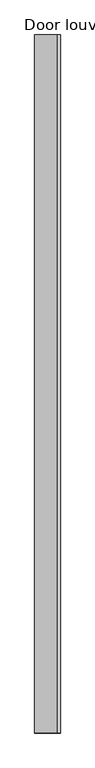
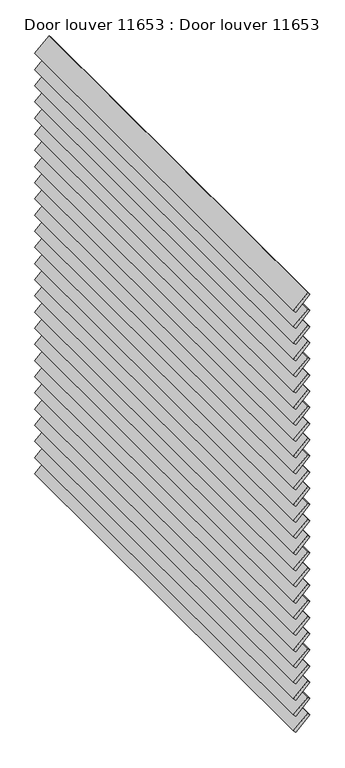
"""IFC4 building model written with IfcOpenShell, lengths in millimetres: proxy geometry, Door louver 11653 : Door louver 11653."""

import ifcopenshell
import ifcopenshell.guid

model = None  # the IFC model being written
_history = None  # IfcOwnerHistory: only IFC2X3 demands one
_inside = {}  # id of a spatial element -> (the spatial element, [elements in it])
_under = {}  # id of a project, library or spatial element -> (it, [spatial elements below it])
_declared = {}  # id of a project -> (the project, [libraries it declares])
_typed = {}  # id of a type object -> (the type object, [elements of that type])
_made_of = {}  # id of a material, layer set ... -> (it, [elements and type objects made of it])


def new_model(schema):
    """Start an empty IFC model of exactly this schema.

    Asked for "IFC4X3", IfcOpenShell would pick the latest addendum, in which some entities
    have other attributes; the version numbers below select the first issue.
    IFC2X3 requires an IfcOwnerHistory on every rooted entity: one is made here for all.
    """
    global model, _history
    if schema == "IFC4X3":
        model = ifcopenshell.file(schema_version=(4, 3, 0, 0))
    else:
        model = ifcopenshell.file(schema=schema)
    _inside.clear()
    _under.clear()
    _declared.clear()
    _typed.clear()
    _made_of.clear()
    _history = None
    if model.schema == "IFC2X3":
        org = make("IfcOrganization", Name="unknown")
        user = make(
            "IfcPersonAndOrganization",
            ThePerson=make("IfcPerson", FamilyName="unknown"),
            TheOrganization=org,
        )
        app = make(
            "IfcApplication",
            ApplicationDeveloper=org,
            Version="unknown",
            ApplicationFullName="unknown",
            ApplicationIdentifier="unknown",
        )
        _history = make(
            "IfcOwnerHistory",
            OwningUser=user,
            OwningApplication=app,
            ChangeAction="ADDED",
            CreationDate=0,
        )
    return model


def make(cls, **values):
    """One entity of the class cls with the attributes given. An attribute that is None is left unset."""
    return model.create_entity(
        cls, **{name: value for name, value in values.items() if value is not None}
    )


def rooted(cls, **values):
    """An entity with a GlobalId (a new one), such as an element, a storey or a relation."""
    return make(cls, GlobalId=ifcopenshell.guid.new(), OwnerHistory=_history, **values)


def si_unit(unit_type, name, prefix=None):
    """IfcSIUnit, for example si_unit("LENGTHUNIT", "METRE", prefix="MILLI")."""
    return make("IfcSIUnit", UnitType=unit_type, Prefix=prefix, Name=name)


def assignment(units):
    """IfcUnitAssignment: the units of a project."""
    return None if units is None else make("IfcUnitAssignment", Units=units)


def point(xyz):
    """IfcCartesianPoint."""
    return None if xyz is None else make("IfcCartesianPoint", Coordinates=xyz)


def direction(xyz):
    """IfcDirection."""
    return None if xyz is None else make("IfcDirection", DirectionRatios=xyz)


def frame(location, z_axis=None, x_axis=None):
    """IfcAxis2Placement3D, a coordinate frame: its origin and axes. An axis left out is left unset."""
    return make(
        "IfcAxis2Placement3D",
        Location=point(location),
        Axis=direction(z_axis),
        RefDirection=direction(x_axis),
    )


def origin():
    """The frame at (0, 0, 0) with its axes left unset."""
    return frame((0.0, 0.0, 0.0))


def place(relative_to, where):
    """IfcLocalPlacement: puts the frame where relative to a parent placement (None: the world)."""
    return make(
        "IfcLocalPlacement", PlacementRelTo=relative_to, RelativePlacement=where
    )


def context(
    kind, dimensions, precision=None, world=None, true_north=None, identifier=None
):
    """IfcGeometricRepresentationContext, for example the 3D "Model" context."""
    return make(
        "IfcGeometricRepresentationContext",
        ContextIdentifier=identifier,
        ContextType=kind,
        CoordinateSpaceDimension=dimensions,
        Precision=precision,
        WorldCoordinateSystem=world,
        TrueNorth=true_north,
    )


def project(units=None, contexts=None):
    """IfcProject with its units and contexts."""
    return rooted(
        "IfcProject",
        Name="project",
        RepresentationContexts=contexts,
        UnitsInContext=assignment(units),
    )


def spatial(cls, under=None, at=None, **own):
    """A site, building, storey or space (cls), placed at a placement, below another one or the project."""
    s = rooted(cls, ObjectPlacement=at, **own)
    if under is not None:
        _under.setdefault(under.id(), (under, []))[1].append(s)
    return s


def polyline(points):
    """IfcPolyline through the points."""
    return make("IfcPolyline", Points=[point(p) for p in points])


def outline(outer, holes=None, kind="AREA"):
    """IfcArbitraryClosedProfileDef: a profile drawn as a closed curve; with holes, ...WithVoids."""
    if holes is None:
        return make("IfcArbitraryClosedProfileDef", ProfileType=kind, OuterCurve=outer)
    return make(
        "IfcArbitraryProfileDefWithVoids",
        ProfileType=kind,
        OuterCurve=outer,
        InnerCurves=holes,
    )


def extrude(swept, where, along, depth):
    """IfcExtrudedAreaSolid: the profile swept, set in the frame where, extruded along a direction by depth."""
    return make(
        "IfcExtrudedAreaSolid",
        SweptArea=swept,
        Position=where,
        ExtrudedDirection=direction(along),
        Depth=depth,
    )


def shape(context_of_items, identifier, shape_type, items):
    """IfcShapeRepresentation: the items that make up one representation, for example the "Body"."""
    return make(
        "IfcShapeRepresentation",
        ContextOfItems=context_of_items,
        RepresentationIdentifier=identifier,
        RepresentationType=shape_type,
        Items=items,
    )


def source(mapping_origin, context_of_items, identifier, shape_type, items):
    """IfcRepresentationMap: a shape defined once, which mapped items show again and again."""
    return make(
        "IfcRepresentationMap",
        MappingOrigin=mapping_origin,
        MappedRepresentation=shape(context_of_items, identifier, shape_type, items),
    )


def transform(
    local_origin,
    x_axis=None,
    y_axis=None,
    z_axis=None,
    scale=None,
    scale2=None,
    scale3=None,
    uniform=True,
):
    """IfcCartesianTransformationOperator3D, or its non-uniform kind. x_axis, y_axis, z_axis: its Axis1, 2, 3."""
    if uniform:
        return make(
            "IfcCartesianTransformationOperator3D",
            Axis1=direction(x_axis),
            Axis2=direction(y_axis),
            LocalOrigin=point(local_origin),
            Scale=scale,
            Axis3=direction(z_axis),
        )
    return make(
        "IfcCartesianTransformationOperator3DnonUniform",
        Axis1=direction(x_axis),
        Axis2=direction(y_axis),
        LocalOrigin=point(local_origin),
        Scale=scale,
        Axis3=direction(z_axis),
        Scale2=scale2,
        Scale3=scale3,
    )


def mapped(mapping_source, mapping_target):
    """IfcMappedItem: shows the shape of a source again, moved by a transform."""
    return make(
        "IfcMappedItem", MappingSource=mapping_source, MappingTarget=mapping_target
    )


def made_of(thing, what):
    """Note that an element or type object is made of a material, layer set ...; save() writes the relation."""
    if what is not None:
        _made_of.setdefault(what.id(), (what, []))[1].append(thing)
    return thing


def element(
    cls,
    number,
    at=None,
    inside=None,
    cuts=None,
    type_object=None,
    material=None,
    context=None,
    identifier="Body",
    shape_type=None,
    held_by="IfcProductDefinitionShape",
    body=None,
    shapes=None,
    **own,
):
    """One element of the class cls, such as IfcWall. Its Tag is "e" and its number.

    at: its placement. inside: the storey or other place that contains it. cuts: it is an
    opening in that element (IfcRelVoidsElement). A single representation is given by context,
    identifier, shape_type and body (its items); several are given by shapes. held_by: the class
    of the entity that holds the representations. save() writes the other relations.
    """
    e = rooted(cls, Tag="e%d" % number, ObjectPlacement=at, **own)
    if body is not None:
        shapes = [shape(context, identifier, shape_type, body)]
    if shapes is not None:
        e.Representation = make(held_by, Representations=shapes)
    if inside is not None:
        _inside.setdefault(inside.id(), (inside, []))[1].append(e)
    if cuts is not None:
        rooted(
            "IfcRelVoidsElement", RelatingBuildingElement=cuts, RelatedOpeningElement=e
        )
    if type_object is not None:
        _typed.setdefault(type_object.id(), (type_object, []))[1].append(e)
    return made_of(e, material)


def aggregate(whole, parts):
    """IfcRelAggregates: a whole, such as a stair, and the parts it consists of."""
    return rooted("IfcRelAggregates", RelatingObject=whole, RelatedObjects=parts)


def save(model, path):
    """Write the relations noted so far, then the file.

    IfcRelAggregates (storeys below a building ...), IfcRelContainedInSpatialStructure (elements
    in a storey), IfcRelDefinesByType, IfcRelAssociatesMaterial and IfcRelDeclares: one each for
    every whole, place, type object, material and project.
    """
    for whole, parts in _under.values():
        aggregate(whole, parts)
    for where, things in _inside.values():
        rooted(
            "IfcRelContainedInSpatialStructure",
            RelatedElements=things,
            RelatingStructure=where,
        )
    for kind, things in _typed.values():
        rooted("IfcRelDefinesByType", RelatedObjects=things, RelatingType=kind)
    for what, things in _made_of.values():
        rooted("IfcRelAssociatesMaterial", RelatedObjects=things, RelatingMaterial=what)
    for by, libraries in _declared.values():
        rooted("IfcRelDeclares", RelatingContext=by, RelatedDefinitions=libraries)
    model.write(path)


def door_louver_11653_door_louver_11653_7676acec(model_context):
    return source(origin(), model_context, "Body", "SweptSolid", [
        extrude(outline(polyline([(0.0, -88.6), (0.0, 0.0), (2000.0, 0.0), (2000.0, -88.6), (0.0, -88.6)])), frame((-8304.3306423, 6540.4513244, 32854.8547367), z_axis=(-0.6925092278135618, 0.0, 0.721409016711785), x_axis=(0.0, -1.0, 0.0)), (0.0, 0.0, 1.0), 13.8216714),
        extrude(outline(polyline([(0.0, -88.6), (0.0, 0.0), (2000.0, 0.0), (2000.0, -88.6), (0.0, -88.6)])), frame((-8304.3306423, 6540.4513244, 32931.0547367), z_axis=(-0.6925092278135618, 0.0, 0.721409016711785), x_axis=(0.0, -1.0, 0.0)), (0.0, 0.0, 1.0), 13.8216714),
        extrude(outline(polyline([(0.0, -88.6), (0.0, 0.0), (2000.0, 0.0), (2000.0, -88.6), (0.0, -88.6)])), frame((-8304.3306423, 6540.4513244, 33007.2547367), z_axis=(-0.6925092278135618, 0.0, 0.721409016711785), x_axis=(0.0, -1.0, 0.0)), (0.0, 0.0, 1.0), 13.8216714),
        extrude(outline(polyline([(0.0, -88.6), (0.0, 0.0), (2000.0, 0.0), (2000.0, -88.6), (0.0, -88.6)])), frame((-8304.3306423, 6540.4513244, 33083.4547367), z_axis=(-0.6925092278135618, 0.0, 0.721409016711785), x_axis=(0.0, -1.0, 0.0)), (0.0, 0.0, 1.0), 13.8216714),
        extrude(outline(polyline([(0.0, -88.6), (0.0, 0.0), (2000.0, 0.0), (2000.0, -88.6), (0.0, -88.6)])), frame((-8304.3306423, 6540.4513244, 33159.6547367), z_axis=(-0.6925092278135618, 0.0, 0.721409016711785), x_axis=(0.0, -1.0, 0.0)), (0.0, 0.0, 1.0), 13.8216714),
        extrude(outline(polyline([(0.0, -88.6), (0.0, 0.0), (2000.0, 0.0), (2000.0, -88.6), (0.0, -88.6)])), frame((-8304.3306423, 6540.4513244, 33235.8547367), z_axis=(-0.6925092278135618, 0.0, 0.721409016711785), x_axis=(0.0, -1.0, 0.0)), (0.0, 0.0, 1.0), 13.8216714),
        extrude(outline(polyline([(0.0, -88.6), (0.0, 0.0), (2000.0, 0.0), (2000.0, -88.6), (0.0, -88.6)])), frame((-8304.3306423, 6540.4513244, 33312.0547367), z_axis=(-0.6925092278135618, 0.0, 0.721409016711785), x_axis=(0.0, -1.0, 0.0)), (0.0, 0.0, 1.0), 13.8216714),
        extrude(outline(polyline([(0.0, -88.6), (0.0, 0.0), (2000.0, 0.0), (2000.0, -88.6), (0.0, -88.6)])), frame((-8304.3306423, 6540.4513244, 33388.2547367), z_axis=(-0.6925092278135618, 0.0, 0.721409016711785), x_axis=(0.0, -1.0, 0.0)), (0.0, 0.0, 1.0), 13.8216714),
        extrude(outline(polyline([(0.0, -88.6), (0.0, 0.0), (2000.0, 0.0), (2000.0, -88.6), (0.0, -88.6)])), frame((-8304.3306423, 6540.4513244, 33464.4547367), z_axis=(-0.6925092278135618, 0.0, 0.721409016711785), x_axis=(0.0, -1.0, 0.0)), (0.0, 0.0, 1.0), 13.8216714),
        extrude(outline(polyline([(0.0, -88.6), (0.0, 0.0), (2000.0, 0.0), (2000.0, -88.6), (0.0, -88.6)])), frame((-8304.3306423, 6540.4513244, 33540.6547367), z_axis=(-0.6925092278135618, 0.0, 0.721409016711785), x_axis=(0.0, -1.0, 0.0)), (0.0, 0.0, 1.0), 13.8216714),
        extrude(outline(polyline([(0.0, -88.6), (0.0, 0.0), (2000.0, 0.0), (2000.0, -88.6), (0.0, -88.6)])), frame((-8304.3306423, 6540.4513244, 33616.8547367), z_axis=(-0.6925092278135618, 0.0, 0.721409016711785), x_axis=(0.0, -1.0, 0.0)), (0.0, 0.0, 1.0), 13.8216714),
        extrude(outline(polyline([(0.0, -88.6), (0.0, 0.0), (2000.0, 0.0), (2000.0, -88.6), (0.0, -88.6)])), frame((-8304.3306423, 6540.4513244, 33693.0547367), z_axis=(-0.6925092278135618, 0.0, 0.721409016711785), x_axis=(0.0, -1.0, 0.0)), (0.0, 0.0, 1.0), 13.8216714),
        extrude(outline(polyline([(0.0, -88.6), (0.0, 0.0), (2000.0, 0.0), (2000.0, -88.6), (0.0, -88.6)])), frame((-8304.3306423, 6540.4513244, 33769.2547367), z_axis=(-0.6925092278135618, 0.0, 0.721409016711785), x_axis=(0.0, -1.0, 0.0)), (0.0, 0.0, 1.0), 13.8216714),
        extrude(outline(polyline([(0.0, -88.6), (0.0, 0.0), (2000.0, 0.0), (2000.0, -88.6), (0.0, -88.6)])), frame((-8304.3306423, 6540.4513244, 33845.4547367), z_axis=(-0.6925092278135618, 0.0, 0.721409016711785), x_axis=(0.0, -1.0, 0.0)), (0.0, 0.0, 1.0), 13.8216714),
        extrude(outline(polyline([(0.0, -88.6), (0.0, 0.0), (2000.0, 0.0), (2000.0, -88.6), (0.0, -88.6)])), frame((-8304.3306423, 6540.4513244, 33921.6547367), z_axis=(-0.6925092278135618, 0.0, 0.721409016711785), x_axis=(0.0, -1.0, 0.0)), (0.0, 0.0, 1.0), 13.8216714),
        extrude(outline(polyline([(0.0, -88.6), (0.0, 0.0), (2000.0, 0.0), (2000.0, -88.6), (0.0, -88.6)])), frame((-8304.3306423, 6540.4513244, 33997.8547367), z_axis=(-0.6925092278135618, 0.0, 0.721409016711785), x_axis=(0.0, -1.0, 0.0)), (0.0, 0.0, 1.0), 13.8216714),
        extrude(outline(polyline([(0.0, -88.6), (0.0, 0.0), (2000.0, 0.0), (2000.0, -88.6), (0.0, -88.6)])), frame((-8304.3306423, 6540.4513244, 34074.0547367), z_axis=(-0.6925092278135618, 0.0, 0.721409016711785), x_axis=(0.0, -1.0, 0.0)), (0.0, 0.0, 1.0), 13.8216714),
        extrude(outline(polyline([(0.0, -88.6), (0.0, 0.0), (2000.0, 0.0), (2000.0, -88.6), (0.0, -88.6)])), frame((-8304.3306423, 6540.4513244, 34150.2547367), z_axis=(-0.6925092278135618, 0.0, 0.721409016711785), x_axis=(0.0, -1.0, 0.0)), (0.0, 0.0, 1.0), 13.8216714),
        extrude(outline(polyline([(0.0, -88.6), (0.0, 0.0), (2000.0, 0.0), (2000.0, -88.6), (0.0, -88.6)])), frame((-8304.3306423, 6540.4513244, 34226.4547367), z_axis=(-0.6925092278135618, 0.0, 0.721409016711785), x_axis=(0.0, -1.0, 0.0)), (0.0, 0.0, 1.0), 13.8216714),
        extrude(outline(polyline([(0.0, -88.6), (0.0, 0.0), (2000.0, 0.0), (2000.0, -88.6), (0.0, -88.6)])), frame((-8304.3306423, 6540.4513244, 34302.6547367), z_axis=(-0.6925092278135618, 0.0, 0.721409016711785), x_axis=(0.0, -1.0, 0.0)), (0.0, 0.0, 1.0), 13.8216714),
        extrude(outline(polyline([(0.0, -88.6), (0.0, 0.0), (2000.0, 0.0), (2000.0, -88.6), (0.0, -88.6)])), frame((-8304.3306423, 6540.4513244, 34378.8547367), z_axis=(-0.6925092278135618, 0.0, 0.721409016711785), x_axis=(0.0, -1.0, 0.0)), (0.0, 0.0, 1.0), 13.8216714),
        extrude(outline(polyline([(0.0, -88.6), (0.0, 0.0), (2000.0, 0.0), (2000.0, -88.6), (0.0, -88.6)])), frame((-8304.3306423, 6540.4513244, 34455.0547367), z_axis=(-0.6925092278135618, 0.0, 0.721409016711785), x_axis=(0.0, -1.0, 0.0)), (0.0, 0.0, 1.0), 13.8216714),
        extrude(outline(polyline([(0.0, -88.6), (0.0, 0.0), (2000.0, 0.0), (2000.0, -88.6), (0.0, -88.6)])), frame((-8304.3306423, 6540.4513244, 34531.2547367), z_axis=(-0.6925092278135618, 0.0, 0.721409016711785), x_axis=(0.0, -1.0, 0.0)), (0.0, 0.0, 1.0), 13.8216714),
        extrude(outline(polyline([(0.0, -88.6), (0.0, 0.0), (2000.0, 0.0), (2000.0, -88.6), (0.0, -88.6)])), frame((-8304.3306423, 6540.4513244, 34607.4547367), z_axis=(-0.6925092278135618, 0.0, 0.721409016711785), x_axis=(0.0, -1.0, 0.0)), (0.0, 0.0, 1.0), 13.8216714),
        extrude(outline(polyline([(0.0, -88.6), (0.0, 0.0), (2000.0, 0.0), (2000.0, -88.6), (0.0, -88.6)])), frame((-8304.3306423, 6540.4513244, 34683.6547367), z_axis=(-0.6925092278135618, 0.0, 0.721409016711785), x_axis=(0.0, -1.0, 0.0)), (0.0, 0.0, 1.0), 13.8216714),
        extrude(outline(polyline([(0.0, -88.6), (0.0, 0.0), (2000.0, 0.0), (2000.0, -88.6), (0.0, -88.6)])), frame((-8304.3306423, 6540.4513244, 34759.8547367), z_axis=(-0.6925092278135618, 0.0, 0.721409016711785), x_axis=(0.0, -1.0, 0.0)), (0.0, 0.0, 1.0), 13.8216714),
        extrude(outline(polyline([(0.0, -88.6), (0.0, 0.0), (2000.0, 0.0), (2000.0, -88.6), (0.0, -88.6)])), frame((-8304.3306423, 6540.4513244, 34836.0547367), z_axis=(-0.6925092278135618, 0.0, 0.721409016711785), x_axis=(0.0, -1.0, 0.0)), (0.0, 0.0, 1.0), 13.8216714),
    ])


if __name__ == "__main__":
    model = new_model("IFC4")
    model_context = context("Model", 3, world=origin())
    ifc_project = project(units=[si_unit("LENGTHUNIT", "METRE", prefix="MILLI")], contexts=[model_context])
    site = spatial("IfcSite", under=ifc_project)
    building = spatial("IfcBuilding", under=site)
    placement = place(None, origin())
    door_louver_11653_door_louver_11653_shape = door_louver_11653_door_louver_11653_7676acec(model_context)
    element("IfcBuildingElementProxy", 1, Name="Door louver 11653 : Door louver 11653", ObjectType="Door louver 11653 : Door louver 11653", at=placement, inside=building, context=model_context, shape_type="MappedRepresentation", body=[
        mapped(door_louver_11653_door_louver_11653_shape, transform((0.0, 0.0, 0.0), x_axis=(1.0, 0.0, 0.0), y_axis=(0.0, 1.0, 0.0), z_axis=(0.0, 0.0, 1.0))),
    ])
    save(model, "model.ifc")

# Revit data of these elements
# Type "Door louver 11653 : Door louver 11653"
#   NameOverride = "Door louver"
# Element 1 (IfcBuildingElementProxy, "Door louver 11653 : Door louver 11653")
#   Materials on its faces: "WOODEN LOUVERS (SPEC T. B. D.)"
# Materials
#   "WOODEN LOUVERS (SPEC T. B. D.)": class "Unassigned", colour RGB 148 103 60, transparency 0, Cost = 0
